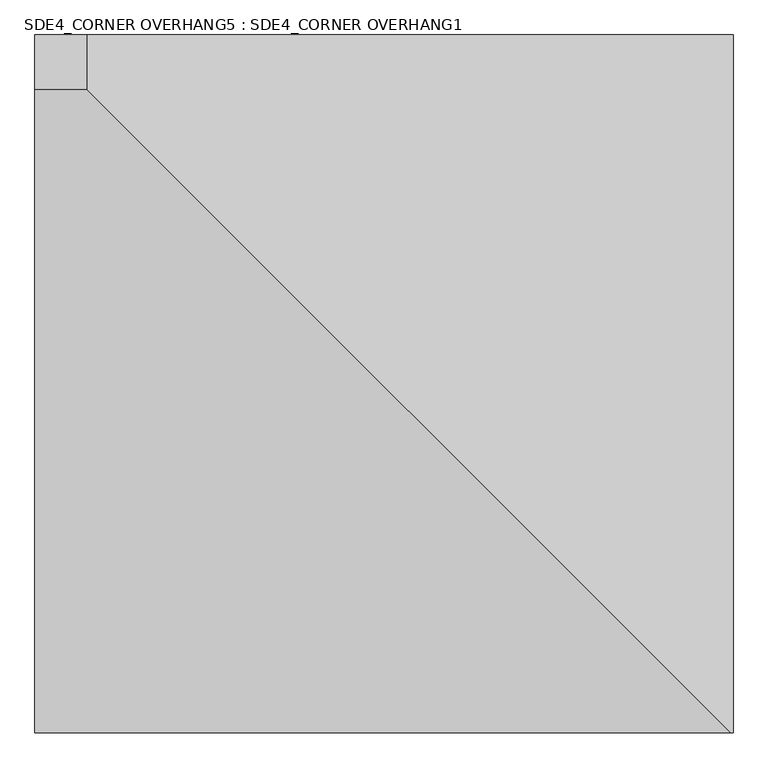
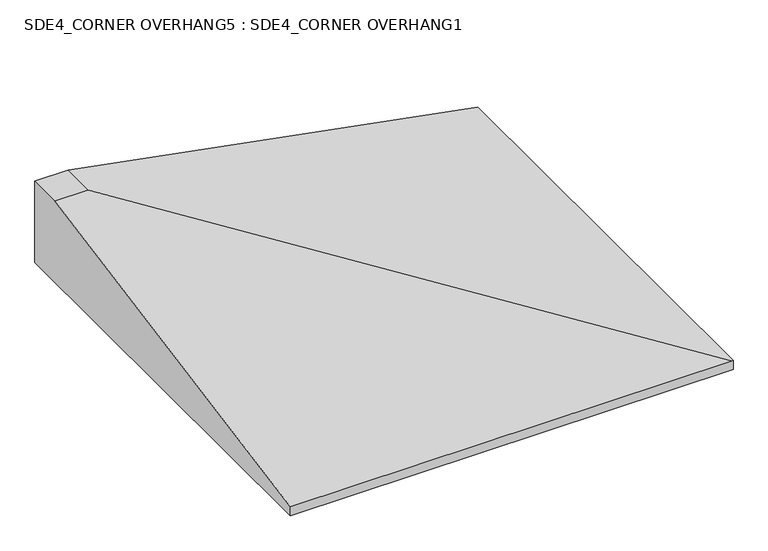
"""IFC4 building model written with IfcOpenShell, lengths in millimetres: proxy geometry, SDE4_CORNER OVERHANG5 : SDE4_CORNER OVERHANG1."""

from ifc_helpers import new_model, si_unit, origin, place, context, project, spatial, faceted_brep, source, transform, mapped, element, save


def sde4_corner_overhang5_sde4_corner_overhang1_667233c2(model_context):
    return source(origin(), model_context, "Body", "Brep", [
        faceted_brep([(71874.3997609, 1190.0524535, 129920.0), (73674.7995218, 1190.0524535, 129920.0), (73674.7995218, 1190.0524535, 129958.8125), (73668.4214976, 1190.0524535, 129960.0), (71874.3997609, 1190.0524535, 129960.0), (72009.7995218, 2990.0524535, 130268.8125), (73674.7995218, 2990.0524535, 129958.8125), (73674.7995218, 2990.0524535, 129920.0), (71874.3997609, 2990.0524535, 129920.0), (71874.3997609, 2990.0524535, 130268.8125), (71874.3997609, 2848.6744293, 130268.8125), (72009.7995218, 2848.6744293, 130268.8125)], [[[0, 1, 2, 3, 4]], [[5, 6, 7, 8, 9]], [[9, 8, 0, 4, 10]], [[1, 0, 8, 7]], [[2, 1, 7, 6]], [[6, 5, 11, 3, 2]], [[4, 3, 11, 10]], [[5, 9, 10, 11]]]),
    ])


if __name__ == "__main__":
    model = new_model("IFC4")
    model_context = context("Model", 3, world=origin())
    ifc_project = project(units=[si_unit("LENGTHUNIT", "METRE", prefix="MILLI")], contexts=[model_context])
    site = spatial("IfcSite", under=ifc_project)
    building = spatial("IfcBuilding", under=site)
    placement = place(None, origin())
    sde4_corner_overhang5_sde4_corner_overhang1_shape = sde4_corner_overhang5_sde4_corner_overhang1_667233c2(model_context)
    element("IfcBuildingElementProxy", 1, Name="SDE4_CORNER OVERHANG5 : SDE4_CORNER OVERHANG1", ObjectType="SDE4_CORNER OVERHANG5 : SDE4_CORNER OVERHANG1", at=placement, inside=building, context=model_context, shape_type="MappedRepresentation", body=[
        mapped(sde4_corner_overhang5_sde4_corner_overhang1_shape, transform((0.0, 0.0, 0.0), x_axis=(1.0, 0.0, 0.0), y_axis=(0.0, 1.0, 0.0), z_axis=(0.0, 0.0, 1.0))),
    ])
    save(model, "model.ifc")
